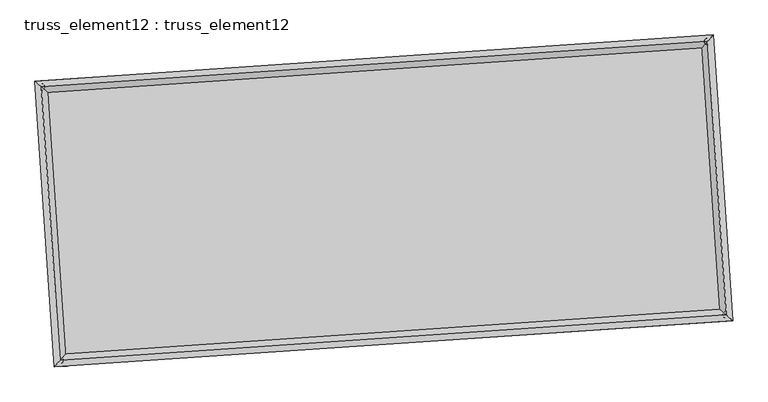
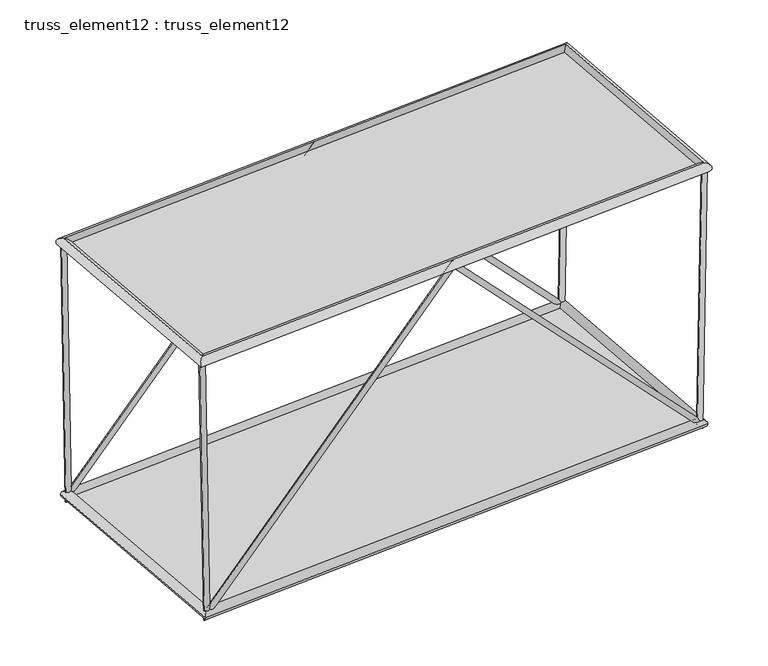
"""IFC4 building model written with IfcOpenShell, lengths in millimetres: plate geometry, truss_element12 : truss_element12."""

import ifcopenshell
import ifcopenshell.guid

model = None  # the IFC model being written
_history = None  # IfcOwnerHistory: only IFC2X3 demands one
_inside = {}  # id of a spatial element -> (the spatial element, [elements in it])
_under = {}  # id of a project, library or spatial element -> (it, [spatial elements below it])
_declared = {}  # id of a project -> (the project, [libraries it declares])
_typed = {}  # id of a type object -> (the type object, [elements of that type])
_made_of = {}  # id of a material, layer set ... -> (it, [elements and type objects made of it])


def new_model(schema):
    """Start an empty IFC model of exactly this schema.

    Asked for "IFC4X3", IfcOpenShell would pick the latest addendum, in which some entities
    have other attributes; the version numbers below select the first issue.
    IFC2X3 requires an IfcOwnerHistory on every rooted entity: one is made here for all.
    """
    global model, _history
    if schema == "IFC4X3":
        model = ifcopenshell.file(schema_version=(4, 3, 0, 0))
    else:
        model = ifcopenshell.file(schema=schema)
    _inside.clear()
    _under.clear()
    _declared.clear()
    _typed.clear()
    _made_of.clear()
    _history = None
    if model.schema == "IFC2X3":
        org = make("IfcOrganization", Name="unknown")
        user = make(
            "IfcPersonAndOrganization",
            ThePerson=make("IfcPerson", FamilyName="unknown"),
            TheOrganization=org,
        )
        app = make(
            "IfcApplication",
            ApplicationDeveloper=org,
            Version="unknown",
            ApplicationFullName="unknown",
            ApplicationIdentifier="unknown",
        )
        _history = make(
            "IfcOwnerHistory",
            OwningUser=user,
            OwningApplication=app,
            ChangeAction="ADDED",
            CreationDate=0,
        )
    return model


def make(cls, **values):
    """One entity of the class cls with the attributes given. An attribute that is None is left unset."""
    return model.create_entity(
        cls, **{name: value for name, value in values.items() if value is not None}
    )


def rooted(cls, **values):
    """An entity with a GlobalId (a new one), such as an element, a storey or a relation."""
    return make(cls, GlobalId=ifcopenshell.guid.new(), OwnerHistory=_history, **values)


def si_unit(unit_type, name, prefix=None):
    """IfcSIUnit, for example si_unit("LENGTHUNIT", "METRE", prefix="MILLI")."""
    return make("IfcSIUnit", UnitType=unit_type, Prefix=prefix, Name=name)


def assignment(units):
    """IfcUnitAssignment: the units of a project."""
    return None if units is None else make("IfcUnitAssignment", Units=units)


def point(xyz):
    """IfcCartesianPoint."""
    return None if xyz is None else make("IfcCartesianPoint", Coordinates=xyz)


def direction(xyz):
    """IfcDirection."""
    return None if xyz is None else make("IfcDirection", DirectionRatios=xyz)


def frame(location, z_axis=None, x_axis=None):
    """IfcAxis2Placement3D, a coordinate frame: its origin and axes. An axis left out is left unset."""
    return make(
        "IfcAxis2Placement3D",
        Location=point(location),
        Axis=direction(z_axis),
        RefDirection=direction(x_axis),
    )


def origin():
    """The frame at (0, 0, 0) with its axes left unset."""
    return frame((0.0, 0.0, 0.0))


def origin_with_axes():
    """The frame at (0, 0, 0) with the z axis (0, 0, 1) and the x axis (1, 0, 0) written out."""
    return frame((0.0, 0.0, 0.0), z_axis=(0.0, 0.0, 1.0), x_axis=(1.0, 0.0, 0.0))


def place(relative_to, where):
    """IfcLocalPlacement: puts the frame where relative to a parent placement (None: the world)."""
    return make(
        "IfcLocalPlacement", PlacementRelTo=relative_to, RelativePlacement=where
    )


def context(
    kind, dimensions, precision=None, world=None, true_north=None, identifier=None
):
    """IfcGeometricRepresentationContext, for example the 3D "Model" context."""
    return make(
        "IfcGeometricRepresentationContext",
        ContextIdentifier=identifier,
        ContextType=kind,
        CoordinateSpaceDimension=dimensions,
        Precision=precision,
        WorldCoordinateSystem=world,
        TrueNorth=true_north,
    )


def project(units=None, contexts=None):
    """IfcProject with its units and contexts."""
    return rooted(
        "IfcProject",
        Name="project",
        RepresentationContexts=contexts,
        UnitsInContext=assignment(units),
    )


def spatial(cls, under=None, at=None, **own):
    """A site, building, storey or space (cls), placed at a placement, below another one or the project."""
    s = rooted(cls, ObjectPlacement=at, **own)
    if under is not None:
        _under.setdefault(under.id(), (under, []))[1].append(s)
    return s


def polyline(points):
    """IfcPolyline through the points."""
    return make("IfcPolyline", Points=[point(p) for p in points])


def circle_curve(where, radius):
    """IfcCircle in the frame where."""
    return make("IfcCircle", Position=where, Radius=radius)


def ellipse_curve(where, semi_axis1, semi_axis2):
    """IfcEllipse in the frame where."""
    return make(
        "IfcEllipse", Position=where, SemiAxis1=semi_axis1, SemiAxis2=semi_axis2
    )


def outline(outer, holes=None, kind="AREA"):
    """IfcArbitraryClosedProfileDef: a profile drawn as a closed curve; with holes, ...WithVoids."""
    if holes is None:
        return make("IfcArbitraryClosedProfileDef", ProfileType=kind, OuterCurve=outer)
    return make(
        "IfcArbitraryProfileDefWithVoids",
        ProfileType=kind,
        OuterCurve=outer,
        InnerCurves=holes,
    )


def extrude(swept, where, along, depth):
    """IfcExtrudedAreaSolid: the profile swept, set in the frame where, extruded along a direction by depth."""
    return make(
        "IfcExtrudedAreaSolid",
        SweptArea=swept,
        Position=where,
        ExtrudedDirection=direction(along),
        Depth=depth,
    )


def shape(context_of_items, identifier, shape_type, items):
    """IfcShapeRepresentation: the items that make up one representation, for example the "Body"."""
    return make(
        "IfcShapeRepresentation",
        ContextOfItems=context_of_items,
        RepresentationIdentifier=identifier,
        RepresentationType=shape_type,
        Items=items,
    )


def source(mapping_origin, context_of_items, identifier, shape_type, items):
    """IfcRepresentationMap: a shape defined once, which mapped items show again and again."""
    return make(
        "IfcRepresentationMap",
        MappingOrigin=mapping_origin,
        MappedRepresentation=shape(context_of_items, identifier, shape_type, items),
    )


def transform(
    local_origin,
    x_axis=None,
    y_axis=None,
    z_axis=None,
    scale=None,
    scale2=None,
    scale3=None,
    uniform=True,
):
    """IfcCartesianTransformationOperator3D, or its non-uniform kind. x_axis, y_axis, z_axis: its Axis1, 2, 3."""
    if uniform:
        return make(
            "IfcCartesianTransformationOperator3D",
            Axis1=direction(x_axis),
            Axis2=direction(y_axis),
            LocalOrigin=point(local_origin),
            Scale=scale,
            Axis3=direction(z_axis),
        )
    return make(
        "IfcCartesianTransformationOperator3DnonUniform",
        Axis1=direction(x_axis),
        Axis2=direction(y_axis),
        LocalOrigin=point(local_origin),
        Scale=scale,
        Axis3=direction(z_axis),
        Scale2=scale2,
        Scale3=scale3,
    )


def mapped(mapping_source, mapping_target):
    """IfcMappedItem: shows the shape of a source again, moved by a transform."""
    return make(
        "IfcMappedItem", MappingSource=mapping_source, MappingTarget=mapping_target
    )


def made_of(thing, what):
    """Note that an element or type object is made of a material, layer set ...; save() writes the relation."""
    if what is not None:
        _made_of.setdefault(what.id(), (what, []))[1].append(thing)
    return thing


def element(
    cls,
    number,
    at=None,
    inside=None,
    cuts=None,
    type_object=None,
    material=None,
    context=None,
    identifier="Body",
    shape_type=None,
    held_by="IfcProductDefinitionShape",
    body=None,
    shapes=None,
    **own,
):
    """One element of the class cls, such as IfcWall. Its Tag is "e" and its number.

    at: its placement. inside: the storey or other place that contains it. cuts: it is an
    opening in that element (IfcRelVoidsElement). A single representation is given by context,
    identifier, shape_type and body (its items); several are given by shapes. held_by: the class
    of the entity that holds the representations. save() writes the other relations.
    """
    e = rooted(cls, Tag="e%d" % number, ObjectPlacement=at, **own)
    if body is not None:
        shapes = [shape(context, identifier, shape_type, body)]
    if shapes is not None:
        e.Representation = make(held_by, Representations=shapes)
    if inside is not None:
        _inside.setdefault(inside.id(), (inside, []))[1].append(e)
    if cuts is not None:
        rooted(
            "IfcRelVoidsElement", RelatingBuildingElement=cuts, RelatedOpeningElement=e
        )
    if type_object is not None:
        _typed.setdefault(type_object.id(), (type_object, []))[1].append(e)
    return made_of(e, material)


def aggregate(whole, parts):
    """IfcRelAggregates: a whole, such as a stair, and the parts it consists of."""
    return rooted("IfcRelAggregates", RelatingObject=whole, RelatedObjects=parts)


def save(model, path):
    """Write the relations noted so far, then the file.

    IfcRelAggregates (storeys below a building ...), IfcRelContainedInSpatialStructure (elements
    in a storey), IfcRelDefinesByType, IfcRelAssociatesMaterial and IfcRelDeclares: one each for
    every whole, place, type object, material and project.
    """
    for whole, parts in _under.values():
        aggregate(whole, parts)
    for where, things in _inside.values():
        rooted(
            "IfcRelContainedInSpatialStructure",
            RelatedElements=things,
            RelatingStructure=where,
        )
    for kind, things in _typed.values():
        rooted("IfcRelDefinesByType", RelatedObjects=things, RelatingType=kind)
    for what, things in _made_of.values():
        rooted("IfcRelAssociatesMaterial", RelatedObjects=things, RelatingMaterial=what)
    for by, libraries in _declared.values():
        rooted("IfcRelDeclares", RelatingContext=by, RelatedDefinitions=libraries)
    model.write(path)


def plane_surface(at):
    """IfcPlane: the flat surface through the origin of the frame at, square to its z axis."""
    return make("IfcPlane", Position=at)


def cylinder_surface(at, radius):
    """IfcCylindricalSurface: all points at the distance radius from the z axis of the frame at."""
    return make("IfcCylindricalSurface", Position=at, Radius=radius)


def advanced_brep(points, edges, surfaces, faces):
    """IfcAdvancedBrep: a solid bounded by faces that lie on surfaces and meet in shared edges.

    An edge is (start, end): straight between two places in points (the first is 0);
    or (start, end, curve); or (start, end, curve, False) where it runs against its curve.
    A face is (place in surfaces, loops), or (place, loops, False) where it looks against
    its surface's normal. A loop lists edges by number (the first is 1), with a minus sign
    where the edge is run from its end to its start. The first loop is the outer one.
    """
    corners = [point(p) for p in points]
    vertices = [make("IfcVertexPoint", VertexGeometry=c) for c in corners]
    made = []
    for start, end, *more in edges:
        made.append(
            make(
                "IfcEdgeCurve",
                EdgeStart=vertices[start],
                EdgeEnd=vertices[end],
                EdgeGeometry=more[0] if more else make("IfcPolyline", Points=[corners[start], corners[end]]),
                SameSense=more[1] if len(more) > 1 else True,
            )
        )
    hull = []
    for where, loops, *sense in faces:
        bounds = []
        for j, loop in enumerate(loops):
            ring = [make("IfcOrientedEdge", EdgeElement=made[abs(k) - 1], Orientation=k > 0) for k in loop]
            bounds.append(
                make(
                    "IfcFaceOuterBound" if j == 0 else "IfcFaceBound",
                    Bound=make("IfcEdgeLoop", EdgeList=ring),
                    Orientation=True,
                )
            )
        hull.append(make("IfcAdvancedFace", Bounds=bounds, FaceSurface=surfaces[where], SameSense=sense[0] if sense else True))
    return make("IfcAdvancedBrep", Outer=make("IfcClosedShell", CfsFaces=hull))


def truss_element12_truss_element12_eb7cdb9d(model_context):
    return source(origin(), model_context, "Body", "SolidModel", [
        advanced_brep(
        [(-3751.912515, 2270.2937696, 5000.1099238), (-3851.0007491, 2256.9335317, 4998.3704092), (-3667.056332, 2276.0797902, 121.9949924), (-3761.9305509, 2263.0068899, -121.9949924), (1063.0047993, 2598.6046781, 5071.3707935), (1063.4636729, 2592.032179, 4927.1341285), (5794.4609613, 2921.2246878, 122.0048162), (5890.3000157, 2921.1558007, -122.0048162), (5877.9325391, 2926.9162974, 5000.120325), (5977.9176694, 2927.1301154, 4998.409186)],
        [
            (0, 1, circle_curve(frame((-3801.4566321, 2263.6136507, 4999.2401665), z_axis=(-0.017392638132463133, -0.0011859378786482353, 0.9998480332981313), x_axis=(-0.13360270549459097, 0.9910343071078557, -0.0011485729311865587)), 50.0)),
            (1, 0, circle_curve(frame((-3801.4566321, 2263.6136507, 4999.2401665), z_axis=(-0.017392638132463133, -0.0011859378786482353, 0.9998480332981313), x_axis=(-0.13360270549459097, 0.9910343071078557, -0.0011485729311865587)), 50.0)),
            (0, 2),
            (2, 3, ellipse_curve(frame((-3714.4934414, 2269.54334, 0.0), z_axis=(-0.9289957394028403, -0.06334468802646137, 0.36462908094418417), x_axis=(0.36378437978405503, 0.024805073983579777, 0.9311528517541036)), 131.300287, 50.0)),
            (3, 1),
            (3, 2, ellipse_curve(frame((-3714.4934414, 2269.54334, 0.0), z_axis=(-0.9289957394028403, -0.06334468802646137, 0.36462908094418417), x_axis=(0.36378437978405503, 0.024805073983579777, 0.9311528517541036)), 131.300287, 50.0)),
            (2, 4),
            (4, 5, ellipse_curve(frame((1063.2342361, 2595.3184285, 4999.252461), z_axis=(-0.9976833933321773, -0.06802823804168447, -7.414941499554083e-05), x_axis=(7.397764016911895e-05, 5.044254070666447e-06, -0.9999999972509321)), 72.2753704, 50.0)),
            (5, 3),
            (5, 4, ellipse_curve(frame((1063.2342361, 2595.3184285, 4999.252461), z_axis=(-0.9976833933321773, -0.06802823804168447, -7.414941499554083e-05), x_axis=(7.397764016911895e-05, 5.044254070666447e-06, -0.9999999972509321)), 72.2753704, 50.0)),
            (4, 6),
            (6, 7, ellipse_curve(frame((5842.3804885, 2921.1902443, 0.0), z_axis=(-0.9289170101606304, -0.06333931977871081, -0.36483053436384116), x_axis=(-0.36398536651592867, -0.02481877850480949, 0.9310739397039283)), 131.3219892, 50.0)),
            (7, 5),
            (7, 6, ellipse_curve(frame((5842.3804885, 2921.1902443, 0.0), z_axis=(-0.9289170101606304, -0.06333931977871081, -0.36483053436384116), x_axis=(-0.36398536651592867, -0.02481877850480949, 0.9310739397039283)), 131.3219892, 50.0)),
            (8, 9, circle_curve(frame((5927.9251043, 2927.0232064, 4999.2647555), z_axis=(0.017108923152044243, 0.001166592432629323, 0.9998529510936464), x_axis=(-0.002157828250047212, 0.9999970336184036, -0.001129836995660202)), 50.0)),
            (9, 8, circle_curve(frame((5927.9251043, 2927.0232064, 4999.2647555), z_axis=(0.017108923152044243, 0.001166592432629323, 0.9998529510936464), x_axis=(-0.002157828250047212, 0.9999970336184036, -0.001129836995660202)), 50.0)),
            (6, 8),
            (9, 7),
        ],
        [
            plane_surface(frame((-3801.4566321, 2313.6136155, 4999.2994724), z_axis=(-0.017392638132462068, -0.0011859378786532565, 0.9998480332981314), x_axis=(0.9998487366290929, -2.0629708890496073e-05, 0.017392625897830513))),
            cylinder_surface(frame((-3801.4566321, 2263.6136507, 4999.2401665), z_axis=(-0.017392638132463136, -0.0011859378786482355, 0.9998480332981315), x_axis=(-0.13360270549459097, 0.9910343071078557, -0.0011485729311865587)), 50.0),
            cylinder_surface(frame((-3714.4934414, 2269.54334, 0.0), z_axis=(-0.6901425550207472, -0.04705819734940098, -0.7221418003492527), x_axis=(-0.020412411512224723, 0.9987523229779233, -0.045575550489902014)), 50.0),
            cylinder_surface(frame((1063.2342361, 2595.3184285, 4999.252461), z_axis=(-0.6902493921239737, -0.047065482165348276, 0.7220392074264583), x_axis=(-0.11534170182495504, 0.9922794555315144, -0.045582605785589675)), 50.0),
            plane_surface(frame((5927.9251043, 2877.0232404, 4999.3230936), z_axis=(0.017108923152043723, 0.0011665924326239086, 0.9998529510936466), x_axis=(0.9998536316624437, -1.9962062093981113e-05, -0.017108911506539936))),
            cylinder_surface(frame((5842.3804885, 2921.1902443, 0.0), z_axis=(-0.017108923152044243, -0.001166592432629323, -0.9998529510936464), x_axis=(-0.002157828250047212, 0.9999970336184036, -0.001129836995660202)), 50.0),
        ],
        [
            (0, [[1, 2]]),
            (1, [[-1, 3, 4, 5]]),
            (1, [[-2, -5, 6, -3]]),
            (2, [[-4, 7, 8, 9]]),
            (2, [[-6, -9, 10, -7]]),
            (3, [[-8, 11, 12, 13]]),
            (3, [[-10, -13, 14, -11]]),
            (4, [[15, 16]]),
            (5, [[-12, 17, -16, 18]]),
            (5, [[-14, -18, -15, -17]]),
        ],
    ),
        advanced_brep(
        [(-3479.7995621, -1720.4398147, 5000.1099238), (-3578.8877962, -1733.8000526, 4998.3704092), (-3394.943379, -1714.6537941, 121.9949924), (-3489.817598, -1727.7266944, -121.9949924), (1335.1177522, -1392.1289062, 5071.3707935), (1335.5766258, -1398.7014053, 4927.1341285), (6066.5739142, -1069.5088965, 122.0048162), (6162.4129686, -1069.5777836, -122.0048162), (6150.045492, -1063.8172869, 5000.120325), (6250.0306223, -1063.6034689, 4998.409186)],
        [
            (0, 1, circle_curve(frame((-3529.3436792, -1727.1199336, 4999.2401665), z_axis=(-0.017392638132463636, -0.0011859378786482945, 0.9998480332981314), x_axis=(-0.1336027054945913, 0.9910343071078556, -0.0011485729311865723)), 50.0)),
            (1, 0, circle_curve(frame((-3529.3436792, -1727.1199336, 4999.2401665), z_axis=(-0.017392638132463636, -0.0011859378786482945, 0.9998480332981314), x_axis=(-0.1336027054945913, 0.9910343071078556, -0.0011485729311865723)), 50.0)),
            (0, 2),
            (2, 3, ellipse_curve(frame((-3442.3804885, -1721.1902443, 0.0), z_axis=(-0.9289957394028405, -0.06334468802646162, 0.3646290809441836), x_axis=(0.3637843797840544, 0.0248050739835798, 0.9311528517541038)), 131.300287, 50.0)),
            (3, 1),
            (3, 2, ellipse_curve(frame((-3442.3804885, -1721.1902443, 0.0), z_axis=(-0.9289957394028405, -0.06334468802646162, 0.3646290809441836), x_axis=(0.3637843797840544, 0.0248050739835798, 0.9311528517541038)), 131.300287, 50.0)),
            (2, 4),
            (4, 5, ellipse_curve(frame((1335.347189, -1395.4151558, 4999.252461), z_axis=(-0.9976833933321773, -0.06802823804168467, -7.414941499586186e-05), x_axis=(7.39776401694264e-05, 5.044254070676052e-06, -0.999999997250932)), 72.2753704, 50.0)),
            (5, 3),
            (5, 4, ellipse_curve(frame((1335.347189, -1395.4151558, 4999.252461), z_axis=(-0.9976833933321773, -0.06802823804168467, -7.414941499586186e-05), x_axis=(7.39776401694264e-05, 5.044254070676052e-06, -0.999999997250932)), 72.2753704, 50.0)),
            (4, 6),
            (6, 7, ellipse_curve(frame((6114.4934414, -1069.54334, 0.0), z_axis=(-0.9289170101606302, -0.063339319778711, -0.3648305343638408), x_axis=(-0.36398536651592855, -0.02481877850480956, 0.9310739397039284)), 131.3219892, 50.0)),
            (7, 5),
            (7, 6, ellipse_curve(frame((6114.4934414, -1069.54334, 0.0), z_axis=(-0.9289170101606302, -0.063339319778711, -0.3648305343638408), x_axis=(-0.36398536651592855, -0.02481877850480956, 0.9310739397039284)), 131.3219892, 50.0)),
            (8, 9, circle_curve(frame((6200.0380572, -1063.7103779, 4999.2647555), z_axis=(0.017108923152044368, 0.0011665924326293448, 0.9998529510936464), x_axis=(-0.0021578282500472473, 0.9999970336184036, -0.001129836995660223)), 50.0)),
            (9, 8, circle_curve(frame((6200.0380572, -1063.7103779, 4999.2647555), z_axis=(0.017108923152044368, 0.0011665924326293448, 0.9998529510936464), x_axis=(-0.0021578282500472473, 0.9999970336184036, -0.001129836995660223)), 50.0)),
            (6, 8),
            (9, 7),
        ],
        [
            plane_surface(frame((-3529.3436792, -1677.1199688, 4999.2994724), z_axis=(-0.017392638132462095, -0.0011859378786532565, 0.9998480332981314), x_axis=(0.9998487366290929, -2.0629708890496107e-05, 0.01739262589783054))),
            cylinder_surface(frame((-3529.3436792, -1727.1199336, 4999.2401665), z_axis=(-0.017392638132463636, -0.0011859378786482945, 0.9998480332981314), x_axis=(-0.1336027054945913, 0.9910343071078556, -0.0011485729311865723)), 50.0),
            cylinder_surface(frame((-3442.3804885, -1721.1902443, 0.0), z_axis=(-0.6901425550207463, -0.047058197349401074, -0.7221418003492535), x_axis=(-0.02041241151222477, 0.9987523229779234, -0.04557555048990207)), 50.0),
            cylinder_surface(frame((1335.347189, -1395.4151558, 4999.252461), z_axis=(-0.6902493921239734, -0.0470654821653484, 0.7220392074264587), x_axis=(-0.11534170182495534, 0.9922794555315144, -0.045582605785589723)), 50.0),
            plane_surface(frame((6200.0380572, -1113.7103439, 4999.3230936), z_axis=(0.017108923152043723, 0.0011665924326347361, 0.9998529510936466), x_axis=(0.9998536316624437, -1.9962062093537024e-05, -0.017108911506539936))),
            cylinder_surface(frame((6114.4934414, -1069.54334, 0.0), z_axis=(-0.017108923152044368, -0.0011665924326293448, -0.9998529510936464), x_axis=(-0.0021578282500472473, 0.9999970336184036, -0.001129836995660223)), 50.0),
        ],
        [
            (0, [[1, 2]]),
            (1, [[-1, 3, 4, 5]]),
            (1, [[-2, -5, 6, -3]]),
            (2, [[-4, 7, 8, 9]]),
            (2, [[-6, -9, 10, -7]]),
            (3, [[-8, 11, 12, 13]]),
            (3, [[-10, -13, 14, -11]]),
            (4, [[15, 16]]),
            (5, [[-12, 17, -16, 18]]),
            (5, [[-14, -18, -15, -17]]),
        ],
    ),
        advanced_brep(
        [(-3529.3372576, -1727.1128164, 4909.2401668), (-3529.3501007, -1727.1270509, 5089.2401662), (-3801.4639603, 2263.6198303, 5089.2401662), (-3801.4493039, 2263.607471, 4909.2401668), (5927.931073, 2927.0302928, 5089.2647552), (5927.9191355, 2927.0161201, 4909.2647557), (6200.0449326, -1063.7165884, 5089.2647552), (6200.0311818, -1063.7041673, 4909.2647557)],
        [
            (0, 1, ellipse_curve(frame((-3529.3436792, -1727.1199336, 4999.2401665), z_axis=(-0.7535719234032147, 0.6573654662782344, -1.782924587316493e-06), x_axis=(-0.657365466275839, -0.7535719234053045, -1.782924587316546e-06)), 127.2792206, 90.0)),
            (1, 2),
            (2, 3, ellipse_curve(frame((-3801.4566321, 2263.6136507, 4999.2401665), z_axis=(-0.6573654662758391, -0.7535719234053043, -1.7829245873165833e-06), x_axis=(0.7535719234032147, -0.6573654662782346, 1.7829245873165301e-06)), 127.2792206, 90.0)),
            (3, 0),
            (1, 0, ellipse_curve(frame((-3529.3436792, -1727.1199336, 4999.2401665), z_axis=(-0.7535719234032147, 0.6573654662782344, -1.782924587316493e-06), x_axis=(-0.657365466275839, -0.7535719234053045, -1.782924587316546e-06)), 127.2792206, 90.0)),
            (3, 2, ellipse_curve(frame((-3801.4566321, 2263.6136507, 4999.2401665), z_axis=(-0.6573654662758391, -0.7535719234053043, -1.7829245873165833e-06), x_axis=(0.7535719234032147, -0.6573654662782346, 1.7829245873165301e-06)), 127.2792206, 90.0)),
            (2, 4),
            (4, 5, ellipse_curve(frame((5927.9251043, 2927.0232064, 4999.2647555), z_axis=(-0.7535719234032134, 0.6573654662782359, -1.7829245873165754e-06), x_axis=(-0.6573654662758406, -0.7535719234053031, -1.782924587316538e-06)), 127.2792206, 90.0)),
            (5, 3),
            (5, 4, ellipse_curve(frame((5927.9251043, 2927.0232064, 4999.2647555), z_axis=(-0.7535719234032134, 0.6573654662782359, -1.7829245873165754e-06), x_axis=(-0.6573654662758406, -0.7535719234053031, -1.782924587316538e-06)), 127.2792206, 90.0)),
            (4, 6),
            (6, 7, ellipse_curve(frame((6200.0380572, -1063.7103779, 4999.2647555), z_axis=(0.6573654662758404, 0.753571923405303, 1.7829245873165003e-06), x_axis=(-0.7535719234032132, 0.6573654662782362, -1.7829245873165377e-06)), 127.2792206, 90.0)),
            (7, 5),
            (7, 6, ellipse_curve(frame((6200.0380572, -1063.7103779, 4999.2647555), z_axis=(0.6573654662758404, 0.753571923405303, 1.7829245873165003e-06), x_axis=(-0.7535719234032132, 0.6573654662782362, -1.7829245873165377e-06)), 127.2792206, 90.0)),
            (6, 1),
            (0, 7),
        ],
        [
            cylinder_surface(frame((-3529.3436792, -1727.1199336, 4999.2401665), z_axis=(0.0680282382287023, -0.9976833960748765, 0.0), x_axis=(-0.997683393150592, -0.06802823802930645, -7.656467492633377e-05)), 90.0),
            cylinder_surface(frame((-3801.4566321, 2263.6136507, 4999.2401665), z_axis=(-0.9976833960717054, -0.06802823822848186, -2.521436132071528e-06), x_axis=(-0.06802823785595627, 0.997683393352727, -7.404323880117403e-05)), 90.0),
            cylinder_surface(frame((5927.9251043, 2927.0232064, 4999.2647555), z_axis=(-0.06802823822869845, 0.9976833960748769, 0.0), x_axis=(0.9976833935231179, 0.0680282380547037, -7.152180267601429e-05)), 90.0),
            cylinder_surface(frame((6200.0380572, -1063.7103779, 4999.2647555), z_axis=(0.9976833960717054, 0.06802823822848189, 2.5214361320714755e-06), x_axis=(0.06802823822848189, -0.9976833933273259, -7.404323880117403e-05)), 90.0),
        ],
        [
            (0, [[1, 2, 3, 4]]),
            (0, [[5, -4, 6, -2]]),
            (1, [[-3, 7, 8, 9]]),
            (1, [[-6, -9, 10, -7]]),
            (2, [[-8, 11, 12, 13]]),
            (2, [[-10, -13, 14, -11]]),
            (3, [[-12, 15, -1, 16]]),
            (3, [[-14, -16, -5, -15]]),
        ],
    ),
        advanced_brep(
        [(-3358.7115243, -1625.2761972, 0.0), (-3526.0494527, -1817.1042913, 0.0), (-3810.4074885, 2353.2123043, 0.0), (-3618.5793943, 2185.8743758, 0.0), (5926.0494527, 3017.1042913, 0.0), (5758.7115243, 2825.2761972, 0.0), (6210.4074885, -1153.2123043, 0.0), (6018.5793943, -985.8743758, 0.0)],
        [
            (0, 1, ellipse_curve(frame((-3442.3804885, -1721.1902443, 0.0), z_axis=(-0.7535719234054579, 0.657365466278081, 0.0), x_axis=(-0.6573654662780811, -0.7535719234054578, 0.0)), 127.2792206, 90.0)),
            (1, 2),
            (2, 3, ellipse_curve(frame((-3714.4934414, 2269.54334, 0.0), z_axis=(-0.6573654662780811, -0.7535719234054578, 0.0), x_axis=(0.7535719234054579, -0.6573654662780809, 0.0)), 127.2792206, 90.0)),
            (3, 0),
            (1, 0, ellipse_curve(frame((-3442.3804885, -1721.1902443, 0.0), z_axis=(-0.7535719234054579, 0.657365466278081, 0.0), x_axis=(-0.6573654662780811, -0.7535719234054578, 0.0)), 127.2792206, 90.0)),
            (3, 2, ellipse_curve(frame((-3714.4934414, 2269.54334, 0.0), z_axis=(-0.6573654662780811, -0.7535719234054578, 0.0), x_axis=(0.7535719234054579, -0.6573654662780809, 0.0)), 127.2792206, 90.0)),
            (2, 4),
            (4, 5, ellipse_curve(frame((5842.3804885, 2921.1902443, 0.0), z_axis=(-0.7535719234054563, 0.6573654662780827, 0.0), x_axis=(-0.6573654662780828, -0.7535719234054563, 0.0)), 127.2792206, 90.0)),
            (5, 3),
            (5, 4, ellipse_curve(frame((5842.3804885, 2921.1902443, 0.0), z_axis=(-0.7535719234054563, 0.6573654662780827, 0.0), x_axis=(-0.6573654662780828, -0.7535719234054563, 0.0)), 127.2792206, 90.0)),
            (4, 6),
            (6, 7, ellipse_curve(frame((6114.4934414, -1069.54334, 0.0), z_axis=(0.6573654662780827, 0.7535719234054564, 0.0), x_axis=(-0.7535719234054565, 0.6573654662780825, 0.0)), 127.2792206, 90.0)),
            (7, 5),
            (7, 6, ellipse_curve(frame((6114.4934414, -1069.54334, 0.0), z_axis=(0.6573654662780827, 0.7535719234054564, 0.0), x_axis=(-0.7535719234054565, 0.6573654662780825, 0.0)), 127.2792206, 90.0)),
            (6, 1),
            (0, 7),
        ],
        [
            cylinder_surface(frame((-3442.3804885, -1721.1902443, 0.0), z_axis=(0.06802823822870294, -0.9976833960748764, 0.0), x_axis=(-0.9976833960748764, -0.06802823822870294, 0.0)), 90.0),
            cylinder_surface(frame((-3714.4934414, 2269.54334, 0.0), z_axis=(-0.9976833960748768, -0.06802823822869876, 0.0), x_axis=(-0.06802823822869876, 0.9976833960748768, 0.0)), 90.0),
            cylinder_surface(frame((5842.3804885, 2921.1902443, 0.0), z_axis=(-0.06802823822869875, 0.9976833960748768, 0.0), x_axis=(0.9976833960748768, 0.06802823822869875, 0.0)), 90.0),
            cylinder_surface(frame((6114.4934414, -1069.54334, 0.0), z_axis=(0.9976833960748768, 0.06802823822869897, 0.0), x_axis=(0.06802823822869897, -0.9976833960748768, 0.0)), 90.0),
        ],
        [
            (0, [[1, 2, 3, 4]]),
            (0, [[5, -4, 6, -2]]),
            (1, [[-3, 7, 8, 9]]),
            (1, [[-6, -9, 10, -7]]),
            (2, [[-8, 11, 12, 13]]),
            (2, [[-10, -13, 14, -11]]),
            (3, [[-12, 15, -1, 16]]),
            (3, [[-14, -16, -5, -15]]),
        ],
    ),
        extrude(outline(polyline([(-3442.3804885, -1721.1902443), (-3714.4934414, 2269.54334), (5842.3804885, 2921.1902443), (6114.4934414, -1069.54334), (-3442.3804885, -1721.1902443)])), origin_with_axes(), (0.0, 0.0, 1.0), 20.0),
        extrude(outline(polyline([(-2000.0, 4875.9865979), (2000.0, 4875.9865978), (2000.0, -4875.986598), (-2000.0, -4875.9865979), (-2000.0, 4875.9865979)])), frame((1199.2907125, 599.9516364, 4999.252461), z_axis=(-2.5155949632309937e-06, -1.7152885787101881e-07, 0.9999999999968213), x_axis=(-0.06802823822870278, 0.9976833960748764, 0.0)), (0.0, 0.0, 1.0), 20.0),
    ])


if __name__ == "__main__":
    model = new_model("IFC4")
    model_context = context("Model", 3, world=origin())
    ifc_project = project(units=[si_unit("LENGTHUNIT", "METRE", prefix="MILLI")], contexts=[model_context])
    site = spatial("IfcSite", under=ifc_project)
    building = spatial("IfcBuilding", under=site)
    placement = place(None, origin())
    truss_element12_truss_element12_shape = truss_element12_truss_element12_eb7cdb9d(model_context)
    element("IfcPlate", 1, ObjectType="truss_element12 : truss_element12", at=placement, inside=building, context=model_context, shape_type="MappedRepresentation", body=[
        mapped(truss_element12_truss_element12_shape, transform((0.0, 0.0, 0.0), x_axis=(1.0, 0.0, 0.0), y_axis=(0.0, 1.0, 0.0), z_axis=(0.0, 0.0, 1.0))),
    ])
    save(model, "model.ifc")

# Revit data of these elements
# Type "truss_element12 : truss_element12"
#   steellbar1 = 90 mm
#   steelbar2 = 50 mm
#   offset1 = 5000 mm
#   M = Default Roof
# Element 1 (IfcPlate, "truss_element12 : truss_element12")
#   Materials on its faces: "Default Roof"
# Materials
#   "Default Roof": class "Miscellaneous", colour RGB 0 127 0, transparency 0, Comments = "Rendering appearance not upgraded Rendering appearance not upgraded ", Cost = 0
